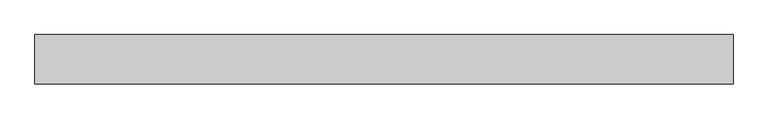
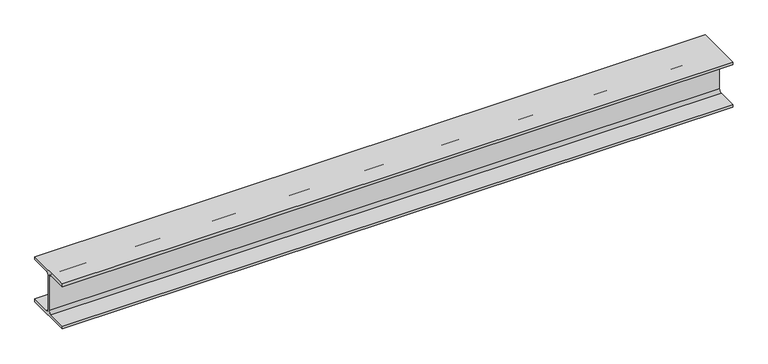
"""IFC4 building model written with IfcOpenShell, lengths in millimetres: beam geometry, 0912_Steel Framing_H-KSD3502 : H_SB_ASB_H-200x200x8x12."""

import ifcopenshell
import ifcopenshell.guid

model = None  # the IFC model being written
_history = None  # IfcOwnerHistory: only IFC2X3 demands one
_inside = {}  # id of a spatial element -> (the spatial element, [elements in it])
_under = {}  # id of a project, library or spatial element -> (it, [spatial elements below it])
_declared = {}  # id of a project -> (the project, [libraries it declares])
_typed = {}  # id of a type object -> (the type object, [elements of that type])
_made_of = {}  # id of a material, layer set ... -> (it, [elements and type objects made of it])


def new_model(schema):
    """Start an empty IFC model of exactly this schema.

    Asked for "IFC4X3", IfcOpenShell would pick the latest addendum, in which some entities
    have other attributes; the version numbers below select the first issue.
    IFC2X3 requires an IfcOwnerHistory on every rooted entity: one is made here for all.
    """
    global model, _history
    if schema == "IFC4X3":
        model = ifcopenshell.file(schema_version=(4, 3, 0, 0))
    else:
        model = ifcopenshell.file(schema=schema)
    _inside.clear()
    _under.clear()
    _declared.clear()
    _typed.clear()
    _made_of.clear()
    _history = None
    if model.schema == "IFC2X3":
        org = make("IfcOrganization", Name="unknown")
        user = make(
            "IfcPersonAndOrganization",
            ThePerson=make("IfcPerson", FamilyName="unknown"),
            TheOrganization=org,
        )
        app = make(
            "IfcApplication",
            ApplicationDeveloper=org,
            Version="unknown",
            ApplicationFullName="unknown",
            ApplicationIdentifier="unknown",
        )
        _history = make(
            "IfcOwnerHistory",
            OwningUser=user,
            OwningApplication=app,
            ChangeAction="ADDED",
            CreationDate=0,
        )
    return model


def make(cls, **values):
    """One entity of the class cls with the attributes given. An attribute that is None is left unset."""
    return model.create_entity(
        cls, **{name: value for name, value in values.items() if value is not None}
    )


def rooted(cls, **values):
    """An entity with a GlobalId (a new one), such as an element, a storey or a relation."""
    return make(cls, GlobalId=ifcopenshell.guid.new(), OwnerHistory=_history, **values)


def si_unit(unit_type, name, prefix=None):
    """IfcSIUnit, for example si_unit("LENGTHUNIT", "METRE", prefix="MILLI")."""
    return make("IfcSIUnit", UnitType=unit_type, Prefix=prefix, Name=name)


def assignment(units):
    """IfcUnitAssignment: the units of a project."""
    return None if units is None else make("IfcUnitAssignment", Units=units)


def point(xyz):
    """IfcCartesianPoint."""
    return None if xyz is None else make("IfcCartesianPoint", Coordinates=xyz)


def direction(xyz):
    """IfcDirection."""
    return None if xyz is None else make("IfcDirection", DirectionRatios=xyz)


def frame(location, z_axis=None, x_axis=None):
    """IfcAxis2Placement3D, a coordinate frame: its origin and axes. An axis left out is left unset."""
    return make(
        "IfcAxis2Placement3D",
        Location=point(location),
        Axis=direction(z_axis),
        RefDirection=direction(x_axis),
    )


def frame_2d(location, x_axis=None):
    """IfcAxis2Placement2D, a coordinate frame in the plane: its origin and x axis."""
    return make(
        "IfcAxis2Placement2D", Location=point(location), RefDirection=direction(x_axis)
    )


def origin():
    """The frame at (0, 0, 0) with its axes left unset."""
    return frame((0.0, 0.0, 0.0))


def place(relative_to, where):
    """IfcLocalPlacement: puts the frame where relative to a parent placement (None: the world)."""
    return make(
        "IfcLocalPlacement", PlacementRelTo=relative_to, RelativePlacement=where
    )


def context(
    kind, dimensions, precision=None, world=None, true_north=None, identifier=None
):
    """IfcGeometricRepresentationContext, for example the 3D "Model" context."""
    return make(
        "IfcGeometricRepresentationContext",
        ContextIdentifier=identifier,
        ContextType=kind,
        CoordinateSpaceDimension=dimensions,
        Precision=precision,
        WorldCoordinateSystem=world,
        TrueNorth=true_north,
    )


def project(units=None, contexts=None):
    """IfcProject with its units and contexts."""
    return rooted(
        "IfcProject",
        Name="project",
        RepresentationContexts=contexts,
        UnitsInContext=assignment(units),
    )


def spatial(cls, under=None, at=None, **own):
    """A site, building, storey or space (cls), placed at a placement, below another one or the project."""
    s = rooted(cls, ObjectPlacement=at, **own)
    if under is not None:
        _under.setdefault(under.id(), (under, []))[1].append(s)
    return s


def polyline(points):
    """IfcPolyline through the points."""
    return make("IfcPolyline", Points=[point(p) for p in points])


def circle_curve(where, radius):
    """IfcCircle in the frame where."""
    return make("IfcCircle", Position=where, Radius=radius)


def trimmed(basis, trim1, trim2, sense, master):
    """IfcTrimmedCurve: the piece of a basis curve between two trims."""
    return make(
        "IfcTrimmedCurve",
        BasisCurve=basis,
        Trim1=trim1,
        Trim2=trim2,
        SenseAgreement=sense,
        MasterRepresentation=master,
    )


def segment(curve, same_sense, transition):
    """IfcCompositeCurveSegment."""
    return make(
        "IfcCompositeCurveSegment",
        Transition=transition,
        SameSense=same_sense,
        ParentCurve=curve,
    )


def composite_curve(segments, self_intersect=None):
    """IfcCompositeCurve: segments joined end to end."""
    return make("IfcCompositeCurve", Segments=segments, SelfIntersect=self_intersect)


def outline(outer, holes=None, kind="AREA"):
    """IfcArbitraryClosedProfileDef: a profile drawn as a closed curve; with holes, ...WithVoids."""
    if holes is None:
        return make("IfcArbitraryClosedProfileDef", ProfileType=kind, OuterCurve=outer)
    return make(
        "IfcArbitraryProfileDefWithVoids",
        ProfileType=kind,
        OuterCurve=outer,
        InnerCurves=holes,
    )


def extrude(swept, where, along, depth):
    """IfcExtrudedAreaSolid: the profile swept, set in the frame where, extruded along a direction by depth."""
    return make(
        "IfcExtrudedAreaSolid",
        SweptArea=swept,
        Position=where,
        ExtrudedDirection=direction(along),
        Depth=depth,
    )


def shape(context_of_items, identifier, shape_type, items):
    """IfcShapeRepresentation: the items that make up one representation, for example the "Body"."""
    return make(
        "IfcShapeRepresentation",
        ContextOfItems=context_of_items,
        RepresentationIdentifier=identifier,
        RepresentationType=shape_type,
        Items=items,
    )


def source(mapping_origin, context_of_items, identifier, shape_type, items):
    """IfcRepresentationMap: a shape defined once, which mapped items show again and again."""
    return make(
        "IfcRepresentationMap",
        MappingOrigin=mapping_origin,
        MappedRepresentation=shape(context_of_items, identifier, shape_type, items),
    )


def transform(
    local_origin,
    x_axis=None,
    y_axis=None,
    z_axis=None,
    scale=None,
    scale2=None,
    scale3=None,
    uniform=True,
):
    """IfcCartesianTransformationOperator3D, or its non-uniform kind. x_axis, y_axis, z_axis: its Axis1, 2, 3."""
    if uniform:
        return make(
            "IfcCartesianTransformationOperator3D",
            Axis1=direction(x_axis),
            Axis2=direction(y_axis),
            LocalOrigin=point(local_origin),
            Scale=scale,
            Axis3=direction(z_axis),
        )
    return make(
        "IfcCartesianTransformationOperator3DnonUniform",
        Axis1=direction(x_axis),
        Axis2=direction(y_axis),
        LocalOrigin=point(local_origin),
        Scale=scale,
        Axis3=direction(z_axis),
        Scale2=scale2,
        Scale3=scale3,
    )


def mapped(mapping_source, mapping_target):
    """IfcMappedItem: shows the shape of a source again, moved by a transform."""
    return make(
        "IfcMappedItem", MappingSource=mapping_source, MappingTarget=mapping_target
    )


def made_of(thing, what):
    """Note that an element or type object is made of a material, layer set ...; save() writes the relation."""
    if what is not None:
        _made_of.setdefault(what.id(), (what, []))[1].append(thing)
    return thing


def element(
    cls,
    number,
    at=None,
    inside=None,
    cuts=None,
    type_object=None,
    material=None,
    context=None,
    identifier="Body",
    shape_type=None,
    held_by="IfcProductDefinitionShape",
    body=None,
    shapes=None,
    **own,
):
    """One element of the class cls, such as IfcWall. Its Tag is "e" and its number.

    at: its placement. inside: the storey or other place that contains it. cuts: it is an
    opening in that element (IfcRelVoidsElement). A single representation is given by context,
    identifier, shape_type and body (its items); several are given by shapes. held_by: the class
    of the entity that holds the representations. save() writes the other relations.
    """
    e = rooted(cls, Tag="e%d" % number, ObjectPlacement=at, **own)
    if body is not None:
        shapes = [shape(context, identifier, shape_type, body)]
    if shapes is not None:
        e.Representation = make(held_by, Representations=shapes)
    if inside is not None:
        _inside.setdefault(inside.id(), (inside, []))[1].append(e)
    if cuts is not None:
        rooted(
            "IfcRelVoidsElement", RelatingBuildingElement=cuts, RelatedOpeningElement=e
        )
    if type_object is not None:
        _typed.setdefault(type_object.id(), (type_object, []))[1].append(e)
    return made_of(e, material)


def aggregate(whole, parts):
    """IfcRelAggregates: a whole, such as a stair, and the parts it consists of."""
    return rooted("IfcRelAggregates", RelatingObject=whole, RelatedObjects=parts)


def save(model, path):
    """Write the relations noted so far, then the file.

    IfcRelAggregates (storeys below a building ...), IfcRelContainedInSpatialStructure (elements
    in a storey), IfcRelDefinesByType, IfcRelAssociatesMaterial and IfcRelDeclares: one each for
    every whole, place, type object, material and project.
    """
    for whole, parts in _under.values():
        aggregate(whole, parts)
    for where, things in _inside.values():
        rooted(
            "IfcRelContainedInSpatialStructure",
            RelatedElements=things,
            RelatingStructure=where,
        )
    for kind, things in _typed.values():
        rooted("IfcRelDefinesByType", RelatedObjects=things, RelatingType=kind)
    for what, things in _made_of.values():
        rooted("IfcRelAssociatesMaterial", RelatedObjects=things, RelatingMaterial=what)
    for by, libraries in _declared.values():
        rooted("IfcRelDeclares", RelatingContext=by, RelatedDefinitions=libraries)
    model.write(path)


def beam_015ba6da(model_context):
    return source(origin(), model_context, "Body", "SweptSolid", [
        extrude(outline(composite_curve([segment(polyline([(100.0, -88.0), (100.0, -100.0), (-100.0, -100.0), (-100.0, -88.0), (-17.0, -88.0)]), True, "CONTINUOUS"), segment(trimmed(circle_curve(frame_2d((-17.0, -75.0)), 13.0), [point((-17.0, -88.0))], [point((-4.0, -75.0))], True, "CARTESIAN"), True, "CONTINUOUS"), segment(polyline([(-4.0, -75.0), (-4.0, 75.0)]), True, "CONTINUOUS"), segment(trimmed(circle_curve(frame_2d((-17.0, 75.0)), 13.0), [point((-4.0, 75.0))], [point((-17.0, 88.0))], True, "CARTESIAN"), True, "CONTINUOUS"), segment(polyline([(-17.0, 88.0), (-100.0, 88.0), (-100.0, 100.0), (100.0, 100.0), (100.0, 88.0), (17.0, 88.0)]), True, "CONTINUOUS"), segment(trimmed(circle_curve(frame_2d((17.0, 75.0)), 13.0), [point((17.0, 88.0))], [point((4.0, 75.0))], True, "CARTESIAN"), True, "CONTINUOUS"), segment(polyline([(4.0, 75.0), (4.0, -75.0)]), True, "CONTINUOUS"), segment(trimmed(circle_curve(frame_2d((17.0, -75.0)), 13.0), [point((4.0, -75.0))], [point((17.0, -88.0))], True, "CARTESIAN"), True, "CONTINUOUS"), segment(polyline([(17.0, -88.0), (100.0, -88.0)]), True, "CONTINUOUS")], self_intersect=False)), frame((-1249.4797233, 0.0, 0.0), z_axis=(1.0, 0.0, 0.0), x_axis=(0.0, 1.0, 0.0)), (0.0, 0.0, 1.0), 2817.4800203),
    ])


if __name__ == "__main__":
    model = new_model("IFC4")
    model_context = context("Model", 3, world=origin())
    ifc_project = project(units=[si_unit("LENGTHUNIT", "METRE", prefix="MILLI")], contexts=[model_context])
    site = spatial("IfcSite", under=ifc_project)
    building = spatial("IfcBuilding", under=site)
    placement = place(None, origin())
    beam_shape = beam_015ba6da(model_context)
    element("IfcBeam", 1, ObjectType="0912_Steel Framing_H-KSD3502 : H_SB_ASB_H-200x200x8x12", at=placement, inside=building, context=model_context, shape_type="MappedRepresentation", body=[
        mapped(beam_shape, transform((0.0, 0.0, 0.0), x_axis=(1.0, 0.0, 0.0), y_axis=(0.0, 1.0, 0.0), z_axis=(0.0, 0.0, 1.0))),
    ])
    save(model, "model.ifc")

# Revit data of these elements
# Type "0912_Steel Framing_H-KSD3502 : H_SB_ASB_H-200x200x8x12"
#   H_WM Code_1 = "S01AA002-00001 | Main Steel Structure Fabrication Work | Shelter/Building | Medium Steel - Standard (90KG/M>Weight≥30KG/M) | Material: (   )"
#   H_WM Code_2 = "S03AA028-00001 | Main Steel Structure Erection Work | Shelter/Building | Medium Steel (90KG/M>Weight≥30KG/M) | Material: (   )"
#   H_WM Code_3 = "S01AA010-00001 | Main Steel Structure Fabrication Work | Shelter/Building | Steel Painting/Coating | for Non-Fireproofed Steel Surface, Surface Preparation, Primer, Second & Final Coat | Material: (   )"
#   H_Q'ty Cal Type Tag = "SB-Q2"
#   Width = 20.0 cm
#   Web Thickness = 0.8 cm
#   Web Fillet = 1.3 cm
#   Warping Constant = 141000.0 cm⁶
#   W = 0
#   Torsional Moment of Inertia = 26.2485 cm⁴
#   Section Area = 63.53 cm²
#   Plastic Modulus weak axis = 244.0 cm³
#   Plastic Modulus strong axis = 525.0 cm³
#   Perimeter = 1.16 m²/m
#   Nominal Weight = 49.90 kgf/m
#   Moment of Inertia weak axis = 1600.00 cm⁴
#   Moment of Inertia strong axis = 4720.00 cm⁴
#   Height = 20.0 cm
#   Flange Thickness = 1.2 cm
#   Elastic Modulus weak axis = 160.0 cm³
#   Elastic Modulus strong axis = 472.0 cm³
#   Centroid Vertical = 10.0 cm
#   Centroid Horizontal = 10.0 cm
#   Ix = 47200000
#   Length [instance default] = 1.5240 m
#   Zx = 525000
#   b = 0.2000 m
#   h = 0.2000 m
#   r = 0.0130 m
#   s = 0.0080 m
#   t = 0.0120 m
#   A = 0.006353 m²
#   Structural Material [instance default] = Steel, 45-345
#   Assembly Code = ""
# Element 1 (IfcBeam, "0912_Steel Framing_H-KSD3502 : H_SB_ASB_H-200x200x8x12")
#   Structural Material = none
# Materials
#   "Steel, 45-345": class "Metal", colour RGB 189 187 185, transparency 0, Description = "Steel 345 MPa", Cost = 0
